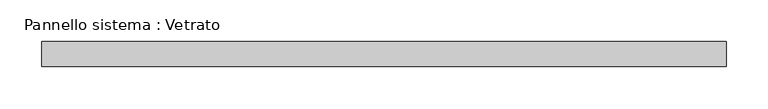
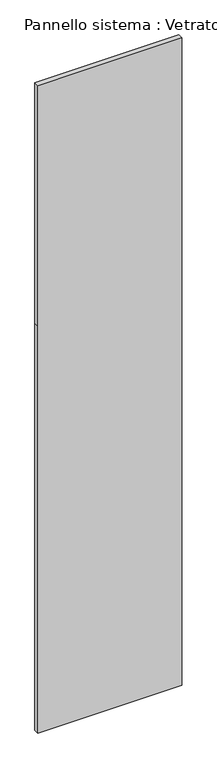
"""IFC4 building model written with IfcOpenShell, lengths in millimetres: plate geometry, Pannello sistema : Vetrato."""

from ifc_helpers import new_model, si_unit, frame, origin, place, context, project, spatial, polyline, outline, extrude, source, transform, mapped, element, save


def pannello_sistema_vetrato_92c996a2(model_context):
    return source(origin(), model_context, "Body", "SweptSolid", [
        extrude(outline(polyline([(0.0, -410.0), (0.0, 410.0), (2450.0, 410.0), (3900.0, 410.0), (3900.0, -410.0), (2450.0, -410.0), (0.0, -410.0)])), frame((0.0, -15.0, 0.0), z_axis=(0.0, 1.0, 0.0), x_axis=(0.0, 0.0, 1.0)), (0.0, 0.0, 1.0), 30.0),
    ])


if __name__ == "__main__":
    model = new_model("IFC4")
    model_context = context("Model", 3, world=origin())
    ifc_project = project(units=[si_unit("LENGTHUNIT", "METRE", prefix="MILLI")], contexts=[model_context])
    site = spatial("IfcSite", under=ifc_project)
    building = spatial("IfcBuilding", under=site)
    placement = place(None, origin())
    pannello_sistema_vetrato_shape = pannello_sistema_vetrato_92c996a2(model_context)
    element("IfcPlate", 1, ObjectType="Pannello sistema : Vetrato", at=placement, inside=building, context=model_context, shape_type="MappedRepresentation", body=[
        mapped(pannello_sistema_vetrato_shape, transform((0.0, 0.0, 0.0), x_axis=(1.0, 0.0, 0.0), y_axis=(0.0, 1.0, 0.0), z_axis=(0.0, 0.0, 1.0))),
    ])
    save(model, "model.ifc")

# Revit data of these elements
# Type "Pannello sistema : Vetrato"
#   Construction Type Id = "GSP4R"
#   Analytic Construction = "Vetrata singola Pilkington 1/8 in"
#   Visual Light Transmittance = 0.9
#   Solar Heat Gain Coefficient = 0.86
#   Heat Transfer Coefficient (U) = 6.7069 W/(m²·K)
# Element 1 (IfcPlate, "Pannello sistema : Vetrato")
#   Materials on its faces: "Default - Vetro"
# Materials
#   "Default - Vetro": class "Vetro", colour RGB 208 208 208, transparency 0.7, Cost = 0
